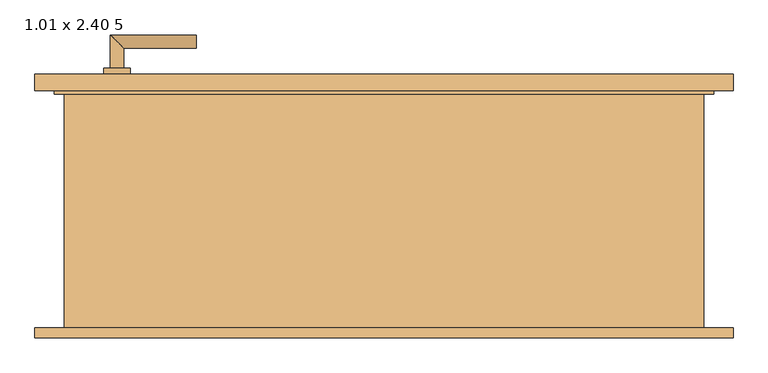
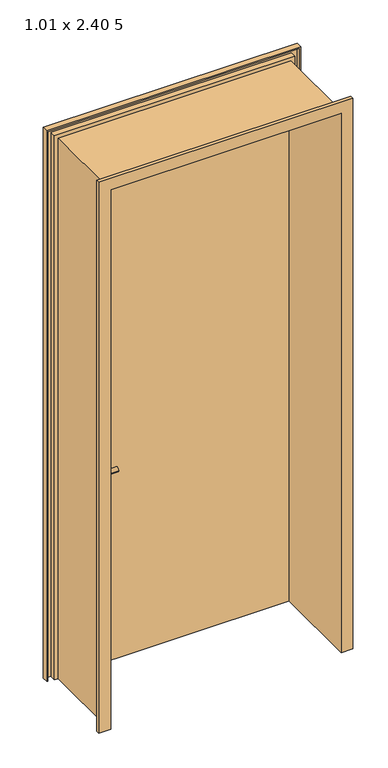
"""IFC4 building model written with IfcOpenShell, lengths in millimetres: door geometry, Drehflügel 1-flg - Stahlzarge : 1.01 x 2.40 5."""

from ifc_helpers import new_model, si_unit, point, frame, frame_2d, origin, place, context, project, spatial, polyline, circle_curve, ellipse_curve, trimmed, segment, composite_curve, outline, extrude, faceted_brep, source, transform, mapped, element, save
from ifc_brep_helpers import plane_surface, cylinder_surface, advanced_brep


def door_1_01_x_2_40_5_82f9e36c(model_context):
    return source(origin(), model_context, "Body", "SolidModel", [
        advanced_brep(
        [(-415.0, 169.4346141, 915.0), (-395.0, 169.4346141, 915.0), (-415.0, 99.4346141, 915.0), (-395.0, 119.4346141, 915.0), (-285.0, 99.4346141, 915.0), (-285.0, 119.4346141, 915.0)],
        [
            (0, 1, circle_curve(frame((-405.0, 169.4346141, 915.0), z_axis=(0.0, 1.0, 0.0), x_axis=(1.0, 0.0, 0.0)), 10.0)),
            (1, 0, circle_curve(frame((-405.0, 169.4346141, 915.0), z_axis=(0.0, 1.0, 0.0), x_axis=(1.0, 0.0, 0.0)), 10.0)),
            (0, 2),
            (2, 3, ellipse_curve(frame((-405.0, 109.4346141, 915.0), z_axis=(-0.7071067811865385, 0.7071067811865565, 0.0), x_axis=(0.7071067811865563, 0.7071067811865386, 0.0)), 14.1421356, 10.0)),
            (3, 1),
            (3, 2, ellipse_curve(frame((-405.0, 109.4346141, 915.0), z_axis=(-0.7071067811865385, 0.7071067811865565, 0.0), x_axis=(0.7071067811865563, 0.7071067811865386, 0.0)), 14.1421356, 10.0)),
            (4, 5, circle_curve(frame((-285.0, 109.4346141, 915.0), z_axis=(1.0, 0.0, 0.0), x_axis=(0.0, 1.0, 0.0)), 10.0)),
            (5, 4, circle_curve(frame((-285.0, 109.4346141, 915.0), z_axis=(1.0, 0.0, 0.0), x_axis=(0.0, 1.0, 0.0)), 10.0)),
            (2, 4),
            (5, 3),
        ],
        [
            plane_surface(frame((-405.0, 169.4346141, -372.7526403), z_axis=(0.0, 1.0, 0.0), x_axis=(0.0, 0.0, 1.0))),
            cylinder_surface(frame((-405.0, 169.4346141, 915.0), z_axis=(0.0, 1.0, 0.0), x_axis=(1.0, 0.0, 0.0)), 10.0),
            plane_surface(frame((-285.0, 109.4346141, -372.7526403), z_axis=(1.0, 0.0, 0.0), x_axis=(0.0, 0.0, 1.0))),
            cylinder_surface(frame((-405.0, 109.4346141, 915.0), z_axis=(-1.0, 0.0, 0.0), x_axis=(0.0, 1.0, 0.0)), 10.0),
        ],
        [
            (0, [[1, 2]]),
            (1, [[-1, 3, 4, 5]]),
            (1, [[-2, -5, 6, -3]]),
            (2, [[7, 8]]),
            (3, [[-4, 9, -8, 10]]),
            (3, [[-6, -10, -7, -9]]),
        ],
    ),
        advanced_brep(
        [(-395.0, 229.4346141, 915.0), (-415.0, 229.4346141, 915.0), (-395.0, 259.4346141, 915.0), (-415.0, 279.4346141, 915.0), (-285.0, 259.4346141, 915.0), (-285.0, 279.4346141, 915.0)],
        [
            (0, 1, circle_curve(frame((-405.0, 229.4346141, 915.0), z_axis=(0.0, -1.0, 0.0), x_axis=(-1.0, 0.0, 0.0)), 10.0)),
            (1, 0, circle_curve(frame((-405.0, 229.4346141, 915.0), z_axis=(0.0, -1.0, 0.0), x_axis=(-1.0, 0.0, 0.0)), 10.0)),
            (0, 2),
            (2, 3, ellipse_curve(frame((-405.0, 269.4346141, 915.0), z_axis=(-0.7071067811865475, -0.7071067811865475, 0.0), x_axis=(0.7071067811865474, -0.7071067811865476, 0.0)), 14.1421356, 10.0)),
            (3, 1),
            (3, 2, ellipse_curve(frame((-405.0, 269.4346141, 915.0), z_axis=(-0.7071067811865475, -0.7071067811865475, 0.0), x_axis=(0.7071067811865474, -0.7071067811865476, 0.0)), 14.1421356, 10.0)),
            (4, 5, circle_curve(frame((-285.0, 269.4346141, 915.0), z_axis=(1.0, 0.0, 0.0), x_axis=(0.0, 1.0, 0.0)), 10.0)),
            (5, 4, circle_curve(frame((-285.0, 269.4346141, 915.0), z_axis=(1.0, 0.0, 0.0), x_axis=(0.0, 1.0, 0.0)), 10.0)),
            (2, 4),
            (5, 3),
        ],
        [
            plane_surface(frame((-405.0, 229.4346141, -372.7526403), z_axis=(0.0, -1.0, 0.0), x_axis=(0.0, 0.0, 1.0))),
            cylinder_surface(frame((-405.0, 229.4346141, 915.0), z_axis=(0.0, -1.0, 0.0), x_axis=(-1.0, 0.0, 0.0)), 10.0),
            plane_surface(frame((-285.0, 269.4346141, -372.7526403), z_axis=(1.0, 0.0, 0.0), x_axis=(0.0, 0.0, 1.0))),
            cylinder_surface(frame((-405.0, 269.4346141, 915.0), z_axis=(-1.0, 0.0, 0.0), x_axis=(0.0, 1.0, 0.0)), 10.0),
        ],
        [
            (0, [[1, 2]]),
            (1, [[-1, 3, 4, 5]]),
            (1, [[-2, -5, 6, -3]]),
            (2, [[7, 8]]),
            (3, [[-4, 9, -8, 10]]),
            (3, [[-6, -10, -7, -9]]),
        ],
    ),
        extrude(outline(composite_curve([segment(trimmed(circle_curve(frame_2d((915.0, -405.0)), 20.0), [point((915.0, -425.0))], [point((915.0, -385.0))], False, "CARTESIAN"), True, "CONTINUOUS"), segment(trimmed(circle_curve(frame_2d((915.0, -405.0)), 20.0), [point((915.0, -385.0))], [point((915.0, -425.0))], False, "CARTESIAN"), True, "CONTINUOUS")], self_intersect=False)), frame((0.0, 159.4346141, 0.0), z_axis=(0.0, 1.0, 0.0), x_axis=(0.0, 0.0, 1.0)), (0.0, 0.0, 1.0), 10.0),
        extrude(outline(composite_curve([segment(trimmed(circle_curve(frame_2d((915.0, -405.0)), 20.0), [point((915.0, -425.0))], [point((915.0, -385.0))], False, "CARTESIAN"), True, "CONTINUOUS"), segment(trimmed(circle_curve(frame_2d((915.0, -405.0)), 20.0), [point((915.0, -385.0))], [point((915.0, -425.0))], False, "CARTESIAN"), True, "CONTINUOUS")], self_intersect=False)), frame((0.0, 219.4346141, 0.0), z_axis=(0.0, 1.0, 0.0), x_axis=(0.0, 0.0, 1.0)), (0.0, 0.0, 1.0), 10.0),
        extrude(outline(polyline([(495.0, 194.4346141), (-495.0, 194.4346141), (-495.0, 219.4346141), (495.0, 219.4346141), (495.0, 194.4346141)])), frame((0.0, 0.0, 15.0), z_axis=(0.0, 0.0, 1.0), x_axis=(1.0, 0.0, 0.0)), (0.0, 0.0, 1.0), 2390.0),
        faceted_brep([(529.4603207, -180.5653859, 15.0), (480.0, -180.5653859, 15.0), (480.0, 194.4346141, 15.0), (495.0, 194.4346141, 15.0), (495.0, 219.4346141, 15.0), (529.4603207, 219.4346141, 15.0), (529.4603207, 194.4346141, 15.0), (524.4603207, 194.4346141, 15.0), (524.4603207, 214.4346141, 15.0), (500.0, 214.4346141, 15.0), (500.0, 189.4346141, 15.0), (485.0, 189.4346141, 15.0), (485.0, -175.5653859, 15.0), (524.4603207, -175.5653859, 15.0), (524.4603207, -165.5653859, 15.0), (529.4603207, -165.5653859, 15.0), (529.4603207, -180.5653859, 2439.4603207), (-529.4603207, -180.5653859, 2439.4603207), (-529.4603207, -180.5653859, 15.0), (-480.0, -180.5653859, 15.0), (-480.0, -180.5653859, 2390.0), (480.0, -180.5653859, 2390.0), (480.0, 194.4346141, 2390.0), (-480.0, 194.4346141, 2390.0), (-480.0, 194.4346141, 15.0), (-495.0, 194.4346141, 15.0), (-495.0, 194.4346141, 2405.0), (495.0, 194.4346141, 2405.0), (495.0, 219.4346141, 2405.0), (-495.0, 219.4346141, 2405.0), (-495.0, 219.4346141, 15.0), (-529.4603207, 219.4346141, 15.0), (-529.4603207, 219.4346141, 2439.4603207), (529.4603207, 219.4346141, 2439.4603207), (529.4603207, 194.4346141, 2439.4603207), (-529.4603207, 194.4346141, 2439.4603207), (-529.4603207, 194.4346141, 15.0), (-524.4603207, 194.4346141, 15.0), (-524.4603207, 194.4346141, 2434.4603207), (524.4603207, 194.4346141, 2434.4603207), (524.4603207, 214.4346141, 2434.4603207), (-524.4603207, 214.4346141, 2434.4603207), (-524.4603207, 214.4346141, 15.0), (-500.0, 214.4346141, 15.0), (-500.0, 214.4346141, 2410.0), (500.0, 214.4346141, 2410.0), (500.0, 189.4346141, 2410.0), (-500.0, 189.4346141, 2410.0), (-500.0, 189.4346141, 15.0), (-485.0, 189.4346141, 15.0), (-485.0, 189.4346141, 2395.0), (485.0, 189.4346141, 2395.0), (485.0, -175.5653859, 2395.0), (-485.0, -175.5653859, 2395.0), (-485.0, -175.5653859, 15.0), (-524.4603207, -175.5653859, 15.0), (-524.4603207, -175.5653859, 2434.4603207), (524.4603207, -175.5653859, 2434.4603207), (524.4603207, -165.5653859, 2434.4603207), (-524.4603207, -165.5653859, 2434.4603207), (-524.4603207, -165.5653859, 15.0), (-529.4603207, -165.5653859, 15.0), (-529.4603207, -165.5653859, 2439.4603207), (529.4603207, -165.5653859, 2439.4603207)], [[[0, 1, 2, 3, 4, 5, 6, 7, 8, 9, 10, 11, 12, 13, 14, 15]], [[1, 0, 16, 17, 18, 19, 20, 21]], [[2, 1, 21, 22]], [[3, 2, 22, 23, 24, 25, 26, 27]], [[4, 3, 27, 28]], [[5, 4, 28, 29, 30, 31, 32, 33]], [[6, 5, 33, 34]], [[7, 6, 34, 35, 36, 37, 38, 39]], [[8, 7, 39, 40]], [[9, 8, 40, 41, 42, 43, 44, 45]], [[10, 9, 45, 46]], [[11, 10, 46, 47, 48, 49, 50, 51]], [[12, 11, 51, 52]], [[13, 12, 52, 53, 54, 55, 56, 57]], [[14, 13, 57, 58]], [[15, 14, 58, 59, 60, 61, 62, 63]], [[0, 15, 63, 16]], [[17, 62, 61, 18]], [[18, 61, 60, 55, 54, 49, 48, 43, 42, 37, 36, 31, 30, 25, 24, 19]], [[23, 20, 19, 24]], [[29, 26, 25, 30]], [[35, 32, 31, 36]], [[41, 38, 37, 42]], [[47, 44, 43, 48]], [[53, 50, 49, 54]], [[59, 56, 55, 60]], [[22, 21, 20, 23]], [[28, 27, 26, 29]], [[34, 33, 32, 35]], [[40, 39, 38, 41]], [[46, 45, 44, 47]], [[52, 51, 50, 53]], [[58, 57, 56, 59]], [[16, 63, 62, 17]]]),
    ])


if __name__ == "__main__":
    model = new_model("IFC4")
    model_context = context("Model", 3, world=origin())
    ifc_project = project(units=[si_unit("LENGTHUNIT", "METRE", prefix="MILLI")], contexts=[model_context])
    site = spatial("IfcSite", under=ifc_project)
    building = spatial("IfcBuilding", under=site)
    placement = place(None, origin())
    door_1_01_x_2_40_5_shape = door_1_01_x_2_40_5_82f9e36c(model_context)
    element("IfcDoor", 1, ObjectType="Drehflügel 1-flg - Stahlzarge : 1.01 x 2.40 5", at=placement, inside=building, context=model_context, shape_type="MappedRepresentation", body=[
        mapped(door_1_01_x_2_40_5_shape, transform((0.0, 0.0, 0.0), x_axis=(1.0, 0.0, 0.0), y_axis=(0.0, 1.0, 0.0), z_axis=(0.0, 0.0, 1.0))),
    ])
    save(model, "model.ifc")

# Revit data of these elements
# Type "Drehflügel 1-flg - Stahlzarge : 1.01 x 2.40 5"
#   Type Mark = "26"
#   Operation = "SingleSwingRight"
#   Keynote = "16.03"
#   Analytic Construction = "Metall"
#   Thermal Resistance (R) = 0.270117 (m²·K)/W
#   Heat Transfer Coefficient (U) = 3.7021 W/(m²·K)
#   Rough Width = 1.010 m
#   Rough Height [instance default] = 2.500 m
#   Höhe Türgriff [instance default] = 0.900 m
#   Height = 2.400 m
#   Fußbodenaufbau [instance default] = 0.100 m
#   Width = 1.010 m
#   Sichtbarkeit Sturzlinien [instance default] = yes
#   Türgriff auswählen [instance default] = element 221079
#   Türgriff [instance default] = none
#   Türflügel [instance default] = none
#   Rahmen/Pfosten [instance default] = Metall - Lackiert - Grau
#   Visual Light Transmittance = 0
#   Solar Heat Gain Coefficient = 0
#   Function = (empty or 0)
#   Wall Closure = (empty or 0)
# Element 1 (IfcDoor, "Drehflügel 1-flg - Stahlzarge : 1.01 x 2.40 5")
#   Rough Height = 2.415 m
#   Fußbodenaufbau = 0.015 m
#   Materials on its faces: "Metall - Lackiert - Grau", "Metall - Chrom", "Holz - Birke"
# Materials
#   "Metall - Lackiert - Grau": class "Farbe 1", colour RGB 98 98 98, transparency 0, Cost = 0
#   "Metall - Chrom": class "Metall", colour RGB 247 247 247, transparency 0, Cost = 0
#   "Holz - Birke": class "Holz", colour RGB 213 164 103, transparency 0, Cost = 0
